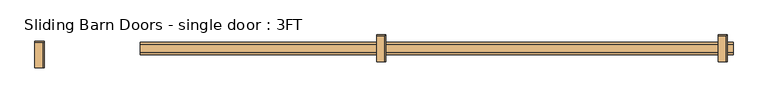
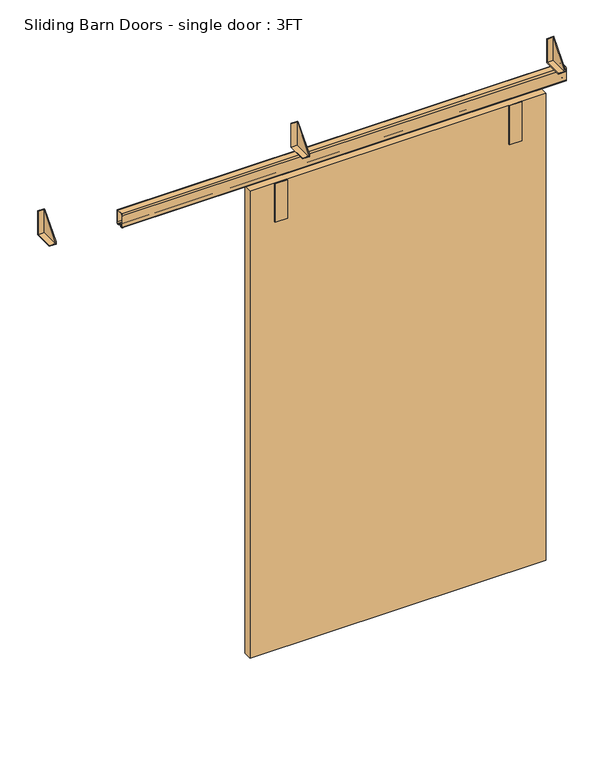
"""IFC4 building model written with IfcOpenShell, lengths in millimetres: door geometry, Sliding Barn Doors - single door : 3FT."""

from ifc_helpers import new_model, si_unit, point, frame, frame_2d, origin, place, context, project, spatial, polyline, circle_curve, trimmed, segment, composite_curve, outline, extrude, source, transform, mapped, element, save


def sliding_barn_doors_single_door_3ft_f1ae4a46(model_context):
    return source(origin(), model_context, "Body", "SweptSolid", [
        extrude(outline(polyline([(-158.75, 2152.65), (-79.375, 2247.773), (-79.375, 2146.3), (-158.75, 2146.3), (-158.75, 2152.65)])), frame((-1538.3371094, 0.0, 0.0), z_axis=(1.0, 0.0, 0.0), x_axis=(0.0, 1.0, 0.0)), (0.0, 0.0, 1.0), 3.175),
        extrude(outline(polyline([(-76.2, 2143.125), (-158.75, 2143.125), (-158.75, 2146.3), (-79.375, 2146.3), (-79.375, 2247.773), (-76.2, 2247.773), (-76.2, 2143.125)])), frame((-1563.6378906, 0.0, 0.0), z_axis=(1.0, 0.0, 0.0), x_axis=(0.0, 1.0, 0.0)), (0.0, 0.0, 1.0), 28.4757812),
        extrude(outline(polyline([(-139.7, 2152.65), (-60.325, 2247.773), (-60.325, 2146.3), (-139.7, 2146.3), (-139.7, 2152.65)])), frame((-484.2371094, 0.0, 0.0), z_axis=(1.0, 0.0, 0.0), x_axis=(0.0, 1.0, 0.0)), (0.0, 0.0, 1.0), 3.175),
        extrude(outline(polyline([(-57.15, 2143.125), (-139.7, 2143.125), (-139.7, 2146.3), (-60.325, 2146.3), (-60.325, 2247.773), (-57.15, 2247.773), (-57.15, 2143.125)])), frame((-509.5378906, 0.0, 0.0), z_axis=(1.0, 0.0, 0.0), x_axis=(0.0, 1.0, 0.0)), (0.0, 0.0, 1.0), 28.4757813),
        extrude(outline(polyline([(-139.7, 2152.65), (-60.325, 2247.773), (-60.325, 2146.3), (-139.7, 2146.3), (-139.7, 2152.65)])), frame((569.8628906, 0.0, 0.0), z_axis=(1.0, 0.0, 0.0), x_axis=(0.0, 1.0, 0.0)), (0.0, 0.0, 1.0), 3.175),
        extrude(outline(polyline([(-57.15, 2143.125), (-139.7, 2143.125), (-139.7, 2146.3), (-60.325, 2146.3), (-60.325, 2247.773), (-57.15, 2247.773), (-57.15, 2143.125)])), frame((544.5621094, 0.0, 0.0), z_axis=(1.0, 0.0, 0.0), x_axis=(0.0, 1.0, 0.0)), (0.0, 0.0, 1.0), 28.4757813),
        extrude(outline(polyline([(-609.854, -117.475), (-609.854, -114.3), (-558.546, -114.3), (-558.546, -117.475), (-609.854, -117.475)])), frame((0.0, 0.0, 1889.252), z_axis=(0.0, 0.0, 1.0), x_axis=(1.0, 0.0, 0.0)), (0.0, 0.0, 1.0), 168.148),
        extrude(outline(polyline([(355.346, -117.475), (355.346, -114.3), (406.654, -114.3), (406.654, -117.475), (355.346, -117.475)])), frame((0.0, 0.0, 1889.252), z_axis=(0.0, 0.0, 1.0), x_axis=(1.0, 0.0, 0.0)), (0.0, 0.0, 1.0), 168.148),
        extrude(outline(polyline([(-711.2, -114.3), (-711.2, -79.375), (508.0, -79.375), (508.0, -114.3), (-711.2, -114.3)])), frame((0.0, 0.0, 25.4), z_axis=(0.0, 0.0, 1.0), x_axis=(1.0, 0.0, 0.0)), (0.0, 0.0, 1.0), 2032.0),
        extrude(outline(composite_curve([segment(trimmed(circle_curve(frame_2d((-85.725, 2136.775)), 6.35), [point((-85.725, 2143.125))], [point((-79.375, 2136.775))], False, "CARTESIAN"), True, "CONTINUOUS"), segment(polyline([(-79.375, 2136.775), (-79.375, 2088.515)]), True, "CONTINUOUS"), segment(trimmed(circle_curve(frame_2d((-85.725, 2088.515)), 6.35), [point((-79.375, 2088.515))], [point((-85.725, 2082.165))], False, "CARTESIAN"), True, "CONTINUOUS"), segment(polyline([(-85.725, 2082.165), (-91.1336853, 2082.165)]), True, "CONTINUOUS"), segment(trimmed(circle_curve(frame_2d((-91.1336853, 2083.7525)), 1.5875), [point((-91.1336853, 2082.165))], [point((-92.6920184, 2083.4495907))], False, "CARTESIAN"), True, "CONTINUOUS"), segment(polyline([(-92.6920184, 2083.4495907), (-94.1175341, 2090.7832331), (-92.6013971, 2090.7832331), (-91.2154749, 2083.6532812), (-85.725, 2083.6532812)]), True, "CONTINUOUS"), segment(trimmed(circle_curve(frame_2d((-85.725, 2088.515)), 4.8617187), [point((-85.725, 2083.6532812))], [point((-80.8632813, 2088.515))], True, "CARTESIAN"), True, "CONTINUOUS"), segment(polyline([(-80.8632813, 2088.515), (-80.8632813, 2136.775)]), True, "CONTINUOUS"), segment(trimmed(circle_curve(frame_2d((-85.725, 2136.775)), 4.8617187), [point((-80.8632813, 2136.775))], [point((-85.725, 2141.6367187))], True, "CARTESIAN"), True, "CONTINUOUS"), segment(polyline([(-85.725, 2141.6367187), (-111.252, 2141.6367187)]), True, "CONTINUOUS"), segment(trimmed(circle_curve(frame_2d((-111.252, 2136.775)), 4.8617187), [point((-111.252, 2141.6367187))], [point((-116.1137188, 2136.775))], True, "CARTESIAN"), True, "CONTINUOUS"), segment(polyline([(-116.1137188, 2136.775), (-116.1137188, 2088.515)]), True, "CONTINUOUS"), segment(trimmed(circle_curve(frame_2d((-111.252, 2088.515)), 4.8617187), [point((-116.1137188, 2088.515))], [point((-111.252, 2083.6532812))], True, "CARTESIAN"), True, "CONTINUOUS"), segment(polyline([(-111.252, 2083.6532812), (-105.7615251, 2083.6532812), (-104.3756029, 2090.7832331), (-102.8594659, 2090.7832331), (-104.2849816, 2083.4495907)]), True, "CONTINUOUS"), segment(trimmed(circle_curve(frame_2d((-105.8433147, 2083.7525)), 1.5875), [point((-104.2849816, 2083.4495907))], [point((-105.8433147, 2082.165))], False, "CARTESIAN"), True, "CONTINUOUS"), segment(polyline([(-105.8433147, 2082.165), (-111.252, 2082.165)]), True, "CONTINUOUS"), segment(trimmed(circle_curve(frame_2d((-111.252, 2088.515)), 6.35), [point((-111.252, 2082.165))], [point((-117.602, 2088.515))], False, "CARTESIAN"), True, "CONTINUOUS"), segment(polyline([(-117.602, 2088.515), (-117.602, 2136.775)]), True, "CONTINUOUS"), segment(trimmed(circle_curve(frame_2d((-111.252, 2136.775)), 6.35), [point((-117.602, 2136.775))], [point((-111.252, 2143.125))], False, "CARTESIAN"), True, "CONTINUOUS"), segment(polyline([(-111.252, 2143.125), (-85.725, 2143.125)]), True, "CONTINUOUS")], self_intersect=False)), frame((-1238.25, 0.0, 0.0), z_axis=(1.0, 0.0, 0.0), x_axis=(0.0, 1.0, 0.0)), (0.0, 0.0, 1.0), 1828.8),
    ])


if __name__ == "__main__":
    model = new_model("IFC4")
    model_context = context("Model", 3, world=origin())
    ifc_project = project(units=[si_unit("LENGTHUNIT", "METRE", prefix="MILLI")], contexts=[model_context])
    site = spatial("IfcSite", under=ifc_project)
    building = spatial("IfcBuilding", under=site)
    placement = place(None, origin())
    sliding_barn_doors_single_door_3ft_shape = sliding_barn_doors_single_door_3ft_f1ae4a46(model_context)
    element("IfcDoor", 1, ObjectType="Sliding Barn Doors - single door : 3FT", at=placement, inside=building, context=model_context, shape_type="MappedRepresentation", body=[
        mapped(sliding_barn_doors_single_door_3ft_shape, transform((0.0, 0.0, 0.0), x_axis=(1.0, 0.0, 0.0), y_axis=(0.0, 1.0, 0.0), z_axis=(0.0, 0.0, 1.0))),
    ])
    save(model, "model.ifc")

# Revit data of these elements
# Type "Sliding Barn Doors - single door : 3FT"
#   Type Mark = "63"
#   Analytic Construction = "<None>"
#   rail_overlap_left = 0' - 5 1/4"
#   rail_length = 6' - 0"
#   overlap_left = 0' - 2"
#   overlap = 0' - 0"
#   bracket_right = 3' - 7"
#   bracket_left = 0' - 4"
#   Thickness = 0' - 1 3/8"
#   Panel Width = 4' - 0"
#   Panel Height = 6' - 8"
#   Gap 2 = 0' - 0 1/2"
#   Gap 1 = 0' - 0 7/8"
#   Frame Projection Ext. = 0' - 1"
#   Frame Projection Int. = 0' - 1"
#   Frame Width = 0' - 3"
#   Height = 6' - 4"
#   Width = 3' - 0"
#   Bracket_offset = 0' - 5"
#   Door_4 = no
#   Door_3 = no
#   Hardware Material = Metal - Aluminum
#   Door Material = Closet_1
#   Function = (empty or 0)
#   Wall Closure = (empty or 0)
# Element 1 (IfcDoor, "Sliding Barn Doors - single door : 3FT")
#   Materials on its faces: "Metal - Aluminum", "Closet_1"
# Materials
#   "Metal - Aluminum": class "Metal", colour RGB 247 247 247, transparency 0
#   "Closet_1": class "Paint", colour RGB 58 62 47, transparency 0, Cost = 0
